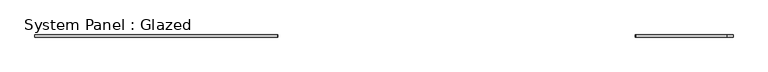
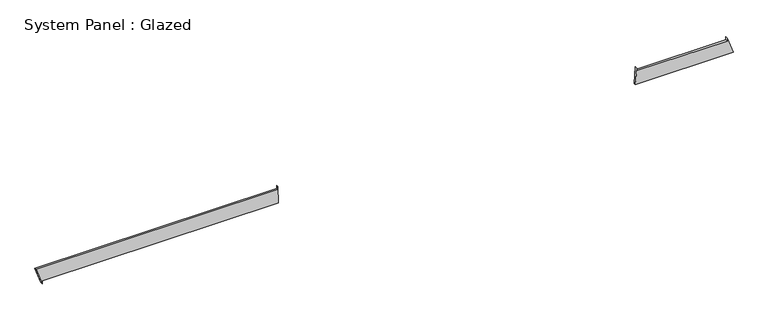
"""IFC4 building model written with IfcOpenShell, lengths in millimetres: plate geometry, System Panel : Glazed."""

from ifc_helpers import new_model, si_unit, frame, origin, place, context, project, spatial, polyline, outline, extrude, source, transform, mapped, element, save


def system_panel_glazed_8d07b756(model_context):
    return source(origin(), model_context, "Body", "SweptSolid", [
        extrude(outline(polyline([(0.0, -3959.0543609), (35.3553391, -3959.0543609), (35.3553391, -1228.347525), (234.7680152, -1233.8641717), (199.4126761, -1233.863729), (199.3776864, -4027.7767133), (0.0, -3959.0543609)])), frame((0.0, -49.5, 0.0), z_axis=(0.0, 1.0, 0.0), x_axis=(0.0, 0.0, 1.0)), (0.0, 0.0, 1.0), 25.0),
        extrude(outline(polyline([(35.3553391, 2899.7253583), (35.3553391, 4027.7767133), (234.8330521, 3959.2965957), (199.477713, 3959.2970385), (199.4646077, 2912.8416231), (234.8199467, 2912.8411803), (35.3553391, 2899.7253583)])), frame((0.0, -49.5, 0.0), z_axis=(0.0, 1.0, 0.0), x_axis=(0.0, 0.0, 1.0)), (0.0, 0.0, 1.0), 25.0),
    ])


if __name__ == "__main__":
    model = new_model("IFC4")
    model_context = context("Model", 3, world=origin())
    ifc_project = project(units=[si_unit("LENGTHUNIT", "METRE", prefix="MILLI")], contexts=[model_context])
    site = spatial("IfcSite", under=ifc_project)
    building = spatial("IfcBuilding", under=site)
    placement = place(None, origin())
    system_panel_glazed_shape = system_panel_glazed_8d07b756(model_context)
    element("IfcPlate", 1, ObjectType="System Panel : Glazed", at=placement, inside=building, context=model_context, shape_type="MappedRepresentation", body=[
        mapped(system_panel_glazed_shape, transform((0.0, 0.0, 0.0), x_axis=(1.0, 0.0, 0.0), y_axis=(0.0, 1.0, 0.0), z_axis=(0.0, 0.0, 1.0))),
    ])
    save(model, "model.ifc")

# Revit data of these elements
# Element 1 (IfcPlate, "System Panel : Glazed")
#   Materials on its faces: "Glass"
# Materials
#   "Glass": class "Glass", colour RGB 218 227 224, transparency 0.85, Description = "Soda Lime Glass", Cost = 0
